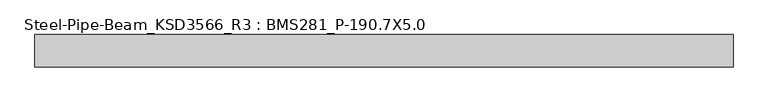
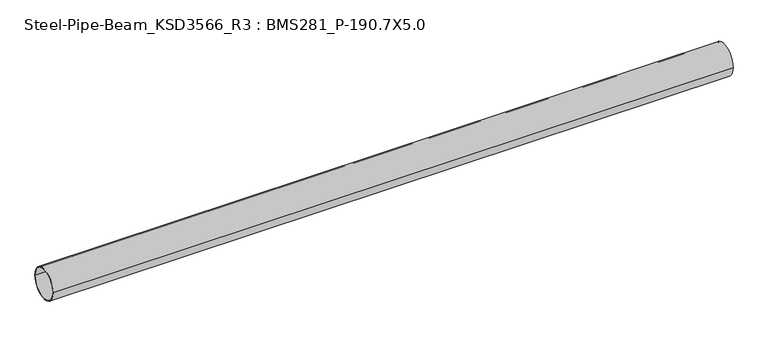
"""IFC4 building model written with IfcOpenShell, lengths in millimetres: member geometry, Steel-Pipe-Beam_KSD3566_R3 : BMS281_P-190.7X5.0."""

from ifc_helpers import new_model, si_unit, point, frame, origin, origin_2d, place, context, project, spatial, circle_curve, trimmed, segment, composite_curve, outline, extrude, source, transform, mapped, element, save


def steel_pipe_beam_ksd3566_r3_bms281_p_190_7x5_0_b754f611(model_context):
    return source(origin(), model_context, "Body", "SweptSolid", [
        extrude(outline(composite_curve([segment(trimmed(circle_curve(origin_2d(), 95.35), [point((-95.35, 0.0))], [point((95.35, 0.0))], False, "CARTESIAN"), True, "CONTINUOUS"), segment(trimmed(circle_curve(origin_2d(), 95.35), [point((95.35, 0.0))], [point((-95.35, 0.0))], False, "CARTESIAN"), True, "CONTINUOUS")], self_intersect=False), holes=[composite_curve([segment(trimmed(circle_curve(origin_2d(), 90.35), [point((90.35, 0.0))], [point((-90.35, 0.0))], True, "CARTESIAN"), True, "CONTINUOUS"), segment(trimmed(circle_curve(origin_2d(), 90.35), [point((-90.35, 0.0))], [point((90.35, 0.0))], True, "CARTESIAN"), True, "CONTINUOUS")], self_intersect=False)]), frame((-2093.8610652, 0.0, 0.0), z_axis=(1.0, 0.0, 0.0), x_axis=(0.0, 1.0, 0.0)), (0.0, 0.0, 1.0), 4122.7134934),
    ])


if __name__ == "__main__":
    model = new_model("IFC4")
    model_context = context("Model", 3, world=origin())
    ifc_project = project(units=[si_unit("LENGTHUNIT", "METRE", prefix="MILLI")], contexts=[model_context])
    site = spatial("IfcSite", under=ifc_project)
    building = spatial("IfcBuilding", under=site)
    placement = place(None, origin())
    steel_pipe_beam_ksd3566_r3_bms281_p_190_7x5_0_shape = steel_pipe_beam_ksd3566_r3_bms281_p_190_7x5_0_b754f611(model_context)
    element("IfcMember", 1, ObjectType="Steel-Pipe-Beam_KSD3566_R3 : BMS281_P-190.7X5.0", at=placement, inside=building, context=model_context, shape_type="MappedRepresentation", body=[
        mapped(steel_pipe_beam_ksd3566_r3_bms281_p_190_7x5_0_shape, transform((0.0, 0.0, 0.0), x_axis=(1.0, 0.0, 0.0), y_axis=(0.0, 1.0, 0.0), z_axis=(0.0, 0.0, 1.0))),
    ])
    save(model, "model.ifc")

# Revit data of these elements
# Type "Steel-Pipe-Beam_KSD3566_R3 : BMS281_P-190.7X5.0"
#   Keynote = "P-190.7X5.0"
#   SteelWeight = "Light"
#   t = 0.0050 m
#   Surface Area = 0.599102 m²/m
#   Section Area = 29.1697 cm²
#   Mass per Unit Length = 22.8982 kg/m
#   Length [instance default] = 1.5000 m
#   D = 0.1907 m
#   hec_material4 [instance default] = none
#   hec_material3 [instance default] = none
#   hec_material2 [instance default] = none
#   hec_material1 [instance default] = none
#   Structural Material [instance default] = Steel, 45-345
#   Assembly Code = ""
# Element 1 (IfcMember, "Steel-Pipe-Beam_KSD3566_R3 : BMS281_P-190.7X5.0")
#   Structural Material = none
# Materials
#   "Steel, 45-345": class "Metal", colour RGB 189 187 185, transparency 0, Description = "Steel 345 MPa", Cost = 0
